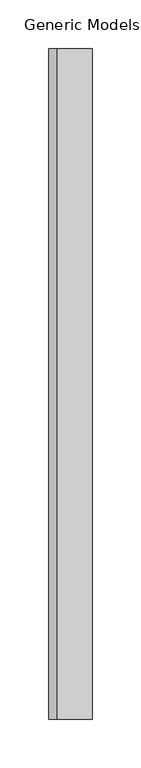
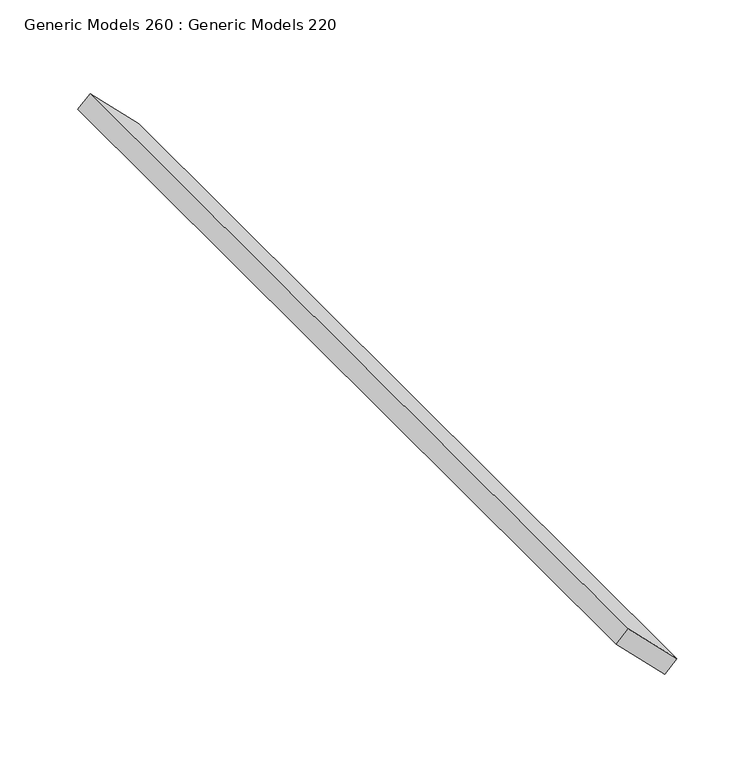
"""IFC4 building model written with IfcOpenShell, lengths in millimetres: proxy geometry, Generic Models 260 : Generic Models 220."""

from ifc_helpers import new_model, si_unit, frame, origin, place, context, project, spatial, polyline, outline, extrude, source, transform, mapped, element, save


def generic_models_260_generic_models_220_1f72fc1b(model_context):
    return source(origin(), model_context, "Body", "SweptSolid", [
        extrude(outline(polyline([(0.0, -50.8), (0.0, 0.0), (690.8142348, 0.0), (690.8142348, -50.8), (0.0, -50.8)])), frame((-6899.085451, -4564.8872686, 128386.6762561), z_axis=(0.7071067811865582, 0.0, 0.7071067811865369), x_axis=(0.0, 1.0, 0.0)), (0.0, 0.0, 1.0), 12.7),
    ])


if __name__ == "__main__":
    model = new_model("IFC4")
    model_context = context("Model", 3, world=origin())
    ifc_project = project(units=[si_unit("LENGTHUNIT", "METRE", prefix="MILLI")], contexts=[model_context])
    site = spatial("IfcSite", under=ifc_project)
    building = spatial("IfcBuilding", under=site)
    placement = place(None, origin())
    generic_models_260_generic_models_220_shape = generic_models_260_generic_models_220_1f72fc1b(model_context)
    element("IfcBuildingElementProxy", 1, Name="Generic Models 260 : Generic Models 220", ObjectType="Generic Models 260 : Generic Models 220", at=placement, inside=building, context=model_context, shape_type="MappedRepresentation", body=[
        mapped(generic_models_260_generic_models_220_shape, transform((0.0, 0.0, 0.0), x_axis=(1.0, 0.0, 0.0), y_axis=(0.0, 1.0, 0.0), z_axis=(0.0, 0.0, 1.0))),
    ])
    save(model, "model.ifc")

# Revit data of these elements
# Element 1 (IfcBuildingElementProxy, "Generic Models 260 : Generic Models 220")
#   Materials on its faces: "_WOOD TONE ALUMINUM EXTRUSION SLAT BY KNOTWOOD"
# Materials
#   "_WOOD TONE ALUMINUM EXTRUSION SLAT BY KNOTWOOD": class "Generic", colour RGB 177 130 114, transparency 0, Cost = 0
